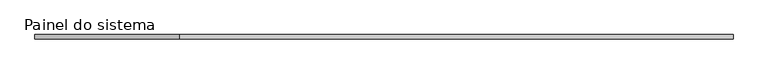
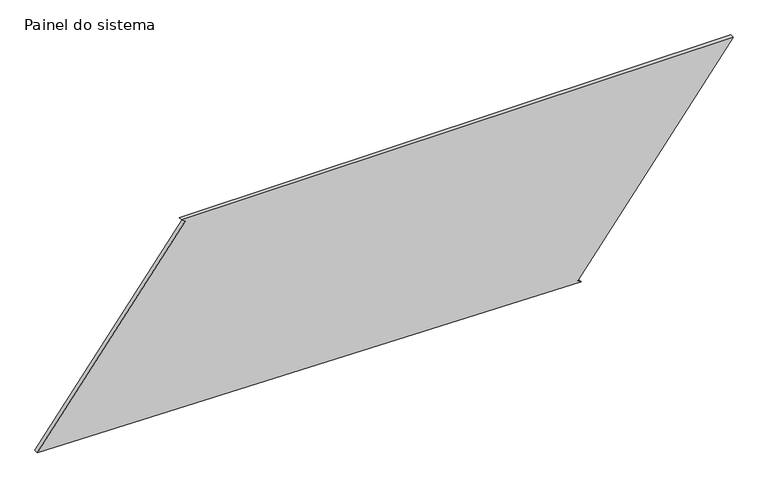
"""IFC4 building model written with IfcOpenShell, lengths in millimetres: plate geometry, Painel do sistema : Envidraçado."""

from ifc_helpers import new_model, si_unit, frame, origin, place, context, project, spatial, polyline, outline, extrude, source, transform, mapped, element, save


def painel_do_sistema_7a3510e2(model_context):
    return source(origin(), model_context, "Body", "SweptSolid", [
        extrude(outline(polyline([(0.0, 1140.0754622), (15.2063352, 1120.2318897), (1195.6116309, 2024.7886931), (1195.6116309, -1184.8512709), (1180.4052957, -1165.0076984), (58.4303844, -2024.7886931), (0.0, 1140.0754622)])), frame((0.0, 24.5, 0.0), z_axis=(0.0, 1.0, 0.0), x_axis=(0.0, 0.0, 1.0)), (0.0, 0.0, 1.0), 25.0),
    ])


if __name__ == "__main__":
    model = new_model("IFC4")
    model_context = context("Model", 3, world=origin())
    ifc_project = project(units=[si_unit("LENGTHUNIT", "METRE", prefix="MILLI")], contexts=[model_context])
    site = spatial("IfcSite", under=ifc_project)
    building = spatial("IfcBuilding", under=site)
    placement = place(None, origin())
    painel_do_sistema_shape = painel_do_sistema_7a3510e2(model_context)
    element("IfcPlate", 1, ObjectType="Painel do sistema : Envidraçado", at=placement, inside=building, context=model_context, shape_type="MappedRepresentation", body=[
        mapped(painel_do_sistema_shape, transform((0.0, 0.0, 0.0), x_axis=(1.0, 0.0, 0.0), y_axis=(0.0, 1.0, 0.0), z_axis=(0.0, 0.0, 1.0))),
    ])
    save(model, "model.ifc")

# Revit data of these elements
# Type "Painel do sistema : Envidraçado"
#   Construction Type Id = "GSP4R"
#   Analytic Construction = "Vidraça única Pilkington 1/8 pol"
#   Visual Light Transmittance = 0.9
#   Solar Heat Gain Coefficient = 0.86
#   Heat Transfer Coefficient (U) = 6.7069 W/(m²·K)
# Element 1 (IfcPlate, "Painel do sistema : Envidraçado")
#   Materials on its faces: "Vidro"
# Materials
#   "Vidro": class "Vidro", colour RGB 0 128 192, transparency 0.9, Description = "Vidro de sílica", Cost = 0
